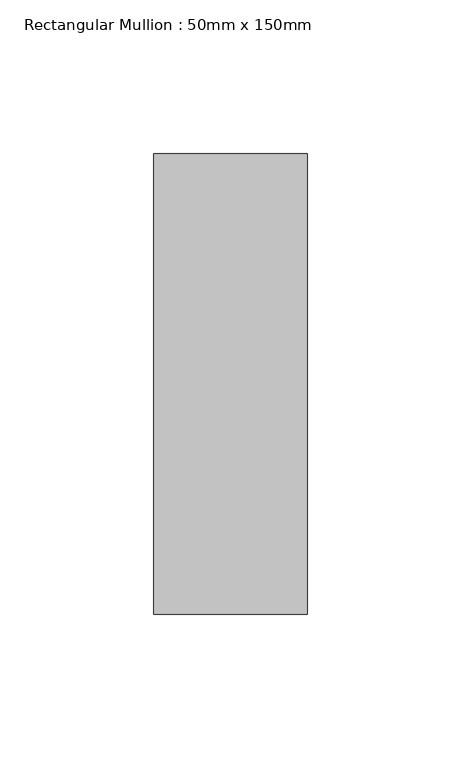
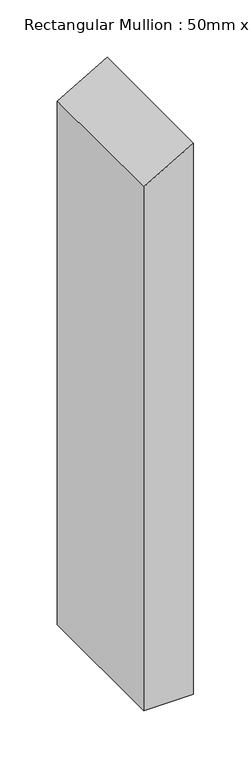
"""IFC4 building model written with IfcOpenShell, lengths in millimetres: member geometry, Rectangular Mullion : 50mm x 150mm."""

from ifc_helpers import new_model, si_unit, frame, origin, place, context, project, spatial, polyline, outline, extrude, source, transform, mapped, element, save


def rectangular_mullion_50mm_x_150mm_450ea858(model_context):
    return source(origin(), model_context, "Body", "SweptSolid", [
        extrude(outline(polyline([(0.0, 0.0), (-28.8675135, -50.0), (-585.6406461, -50.0), (-585.6406461, 0.0), (0.0, 0.0)])), frame((0.0, -75.0, 0.0), z_axis=(0.0, 1.0, 0.0), x_axis=(0.0, 0.0, 1.0)), (0.0, 0.0, 1.0), 150.0),
    ])


if __name__ == "__main__":
    model = new_model("IFC4")
    model_context = context("Model", 3, world=origin())
    ifc_project = project(units=[si_unit("LENGTHUNIT", "METRE", prefix="MILLI")], contexts=[model_context])
    site = spatial("IfcSite", under=ifc_project)
    building = spatial("IfcBuilding", under=site)
    placement = place(None, origin())
    rectangular_mullion_50mm_x_150mm_shape = rectangular_mullion_50mm_x_150mm_450ea858(model_context)
    element("IfcMember", 1, ObjectType="Rectangular Mullion : 50mm x 150mm", at=placement, inside=building, context=model_context, shape_type="MappedRepresentation", body=[
        mapped(rectangular_mullion_50mm_x_150mm_shape, transform((0.0, 0.0, 0.0), x_axis=(1.0, 0.0, 0.0), y_axis=(0.0, 1.0, 0.0), z_axis=(0.0, 0.0, 1.0))),
    ])
    save(model, "model.ifc")

# Revit data of these elements
# Type "Rectangular Mullion : 50mm x 150mm"
#   built-in parameter 1007304 = 0.492126 (stored number, unit not read)
#   built-in parameter 1007301 = 0.082021 (stored number, unit not read)
#   built-in parameter 1007300 = 0.082021 (stored number, unit not read)
# Element 1 (IfcMember, "Rectangular Mullion : 50mm x 150mm")
#   Materials on its faces: "Aluminum"
# Materials
#   "Aluminum": class "Metal", colour RGB 247 247 247, transparency 0, Description = "Aluminum 6061", Cost = 0
